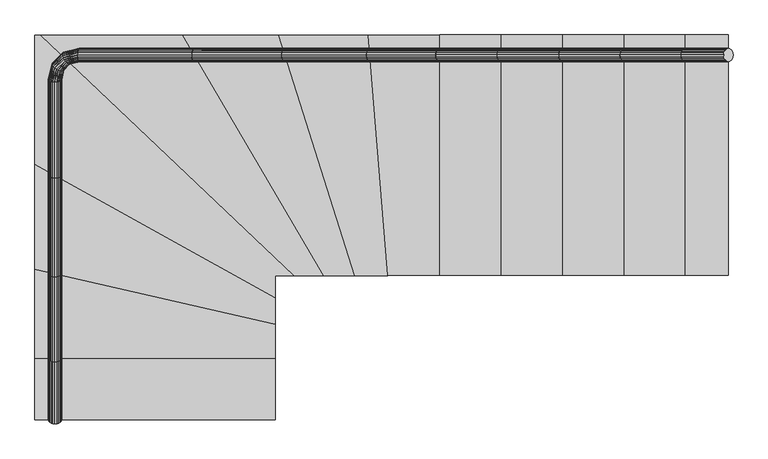
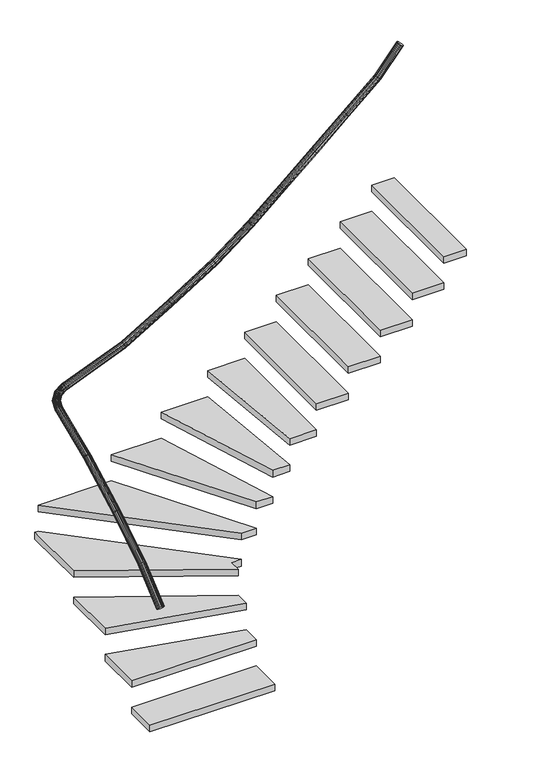
"""IFC4 building model written with IfcOpenShell, lengths in millimetres: stair geometry, 0_3d."""

import ifcopenshell
import ifcopenshell.guid

model = None  # the IFC model being written
_history = None  # IfcOwnerHistory: only IFC2X3 demands one
_inside = {}  # id of a spatial element -> (the spatial element, [elements in it])
_under = {}  # id of a project, library or spatial element -> (it, [spatial elements below it])
_declared = {}  # id of a project -> (the project, [libraries it declares])
_typed = {}  # id of a type object -> (the type object, [elements of that type])
_made_of = {}  # id of a material, layer set ... -> (it, [elements and type objects made of it])


def new_model(schema):
    """Start an empty IFC model of exactly this schema.

    Asked for "IFC4X3", IfcOpenShell would pick the latest addendum, in which some entities
    have other attributes; the version numbers below select the first issue.
    IFC2X3 requires an IfcOwnerHistory on every rooted entity: one is made here for all.
    """
    global model, _history
    if schema == "IFC4X3":
        model = ifcopenshell.file(schema_version=(4, 3, 0, 0))
    else:
        model = ifcopenshell.file(schema=schema)
    _inside.clear()
    _under.clear()
    _declared.clear()
    _typed.clear()
    _made_of.clear()
    _history = None
    if model.schema == "IFC2X3":
        org = make("IfcOrganization", Name="unknown")
        user = make(
            "IfcPersonAndOrganization",
            ThePerson=make("IfcPerson", FamilyName="unknown"),
            TheOrganization=org,
        )
        app = make(
            "IfcApplication",
            ApplicationDeveloper=org,
            Version="unknown",
            ApplicationFullName="unknown",
            ApplicationIdentifier="unknown",
        )
        _history = make(
            "IfcOwnerHistory",
            OwningUser=user,
            OwningApplication=app,
            ChangeAction="ADDED",
            CreationDate=0,
        )
    return model


def make(cls, **values):
    """One entity of the class cls with the attributes given. An attribute that is None is left unset."""
    return model.create_entity(
        cls, **{name: value for name, value in values.items() if value is not None}
    )


def rooted(cls, **values):
    """An entity with a GlobalId (a new one), such as an element, a storey or a relation."""
    return make(cls, GlobalId=ifcopenshell.guid.new(), OwnerHistory=_history, **values)


def si_unit(unit_type, name, prefix=None):
    """IfcSIUnit, for example si_unit("LENGTHUNIT", "METRE", prefix="MILLI")."""
    return make("IfcSIUnit", UnitType=unit_type, Prefix=prefix, Name=name)


def assignment(units):
    """IfcUnitAssignment: the units of a project."""
    return None if units is None else make("IfcUnitAssignment", Units=units)


def point(xyz):
    """IfcCartesianPoint."""
    return None if xyz is None else make("IfcCartesianPoint", Coordinates=xyz)


def direction(xyz):
    """IfcDirection."""
    return None if xyz is None else make("IfcDirection", DirectionRatios=xyz)


def frame(location, z_axis=None, x_axis=None):
    """IfcAxis2Placement3D, a coordinate frame: its origin and axes. An axis left out is left unset."""
    return make(
        "IfcAxis2Placement3D",
        Location=point(location),
        Axis=direction(z_axis),
        RefDirection=direction(x_axis),
    )


def origin():
    """The frame at (0, 0, 0) with its axes left unset."""
    return frame((0.0, 0.0, 0.0))


def origin_with_axes():
    """The frame at (0, 0, 0) with the z axis (0, 0, 1) and the x axis (1, 0, 0) written out."""
    return frame((0.0, 0.0, 0.0), z_axis=(0.0, 0.0, 1.0), x_axis=(1.0, 0.0, 0.0))


def place(relative_to, where):
    """IfcLocalPlacement: puts the frame where relative to a parent placement (None: the world)."""
    return make(
        "IfcLocalPlacement", PlacementRelTo=relative_to, RelativePlacement=where
    )


def context(
    kind, dimensions, precision=None, world=None, true_north=None, identifier=None
):
    """IfcGeometricRepresentationContext, for example the 3D "Model" context."""
    return make(
        "IfcGeometricRepresentationContext",
        ContextIdentifier=identifier,
        ContextType=kind,
        CoordinateSpaceDimension=dimensions,
        Precision=precision,
        WorldCoordinateSystem=world,
        TrueNorth=true_north,
    )


def project(units=None, contexts=None):
    """IfcProject with its units and contexts."""
    return rooted(
        "IfcProject",
        Name="project",
        RepresentationContexts=contexts,
        UnitsInContext=assignment(units),
    )


def spatial(cls, under=None, at=None, **own):
    """A site, building, storey or space (cls), placed at a placement, below another one or the project."""
    s = rooted(cls, ObjectPlacement=at, **own)
    if under is not None:
        _under.setdefault(under.id(), (under, []))[1].append(s)
    return s


def polyline(points):
    """IfcPolyline through the points."""
    return make("IfcPolyline", Points=[point(p) for p in points])


def outline(outer, holes=None, kind="AREA"):
    """IfcArbitraryClosedProfileDef: a profile drawn as a closed curve; with holes, ...WithVoids."""
    if holes is None:
        return make("IfcArbitraryClosedProfileDef", ProfileType=kind, OuterCurve=outer)
    return make(
        "IfcArbitraryProfileDefWithVoids",
        ProfileType=kind,
        OuterCurve=outer,
        InnerCurves=holes,
    )


def extrude(swept, where, along, depth):
    """IfcExtrudedAreaSolid: the profile swept, set in the frame where, extruded along a direction by depth."""
    return make(
        "IfcExtrudedAreaSolid",
        SweptArea=swept,
        Position=where,
        ExtrudedDirection=direction(along),
        Depth=depth,
    )


def faces_of(points, faces, orient=None, outer=None):
    """IfcFace entities. A face is a list of loops; a loop is a list of indices into points, from 0.

    orient and outer hold one flag for each loop. By default every Orientation is true, the
    first loop of a face is its IfcFaceOuterBound and the others are IfcFaceBound.
    """
    made = []
    for i, loops in enumerate(faces):
        bounds = []
        for j, loop in enumerate(loops):
            is_outer = j == 0 if outer is None else outer[i][j]
            bounds.append(
                make(
                    "IfcFaceOuterBound" if is_outer else "IfcFaceBound",
                    Bound=make("IfcPolyLoop", Polygon=[points[k] for k in loop]),
                    Orientation=True if orient is None else orient[i][j],
                )
            )
        made.append(make("IfcFace", Bounds=bounds))
    return made


def faceted_brep(points, faces, orient=None, outer=None, voids=None):
    """IfcFacetedBrep: a solid bounded by flat faces; with voids (closed shells), ...WithVoids."""
    shared = [point(p) for p in points]
    hull = make("IfcClosedShell", CfsFaces=faces_of(shared, faces, orient, outer))
    if voids is None:
        return make("IfcFacetedBrep", Outer=hull)
    return make(
        "IfcFacetedBrepWithVoids",
        Outer=hull,
        Voids=[
            make(cls, CfsFaces=faces_of(shared, fs, o, b)) for cls, fs, o, b in voids
        ],
    )


def shape(context_of_items, identifier, shape_type, items):
    """IfcShapeRepresentation: the items that make up one representation, for example the "Body"."""
    return make(
        "IfcShapeRepresentation",
        ContextOfItems=context_of_items,
        RepresentationIdentifier=identifier,
        RepresentationType=shape_type,
        Items=items,
    )


def source(mapping_origin, context_of_items, identifier, shape_type, items):
    """IfcRepresentationMap: a shape defined once, which mapped items show again and again."""
    return make(
        "IfcRepresentationMap",
        MappingOrigin=mapping_origin,
        MappedRepresentation=shape(context_of_items, identifier, shape_type, items),
    )


def transform(
    local_origin,
    x_axis=None,
    y_axis=None,
    z_axis=None,
    scale=None,
    scale2=None,
    scale3=None,
    uniform=True,
):
    """IfcCartesianTransformationOperator3D, or its non-uniform kind. x_axis, y_axis, z_axis: its Axis1, 2, 3."""
    if uniform:
        return make(
            "IfcCartesianTransformationOperator3D",
            Axis1=direction(x_axis),
            Axis2=direction(y_axis),
            LocalOrigin=point(local_origin),
            Scale=scale,
            Axis3=direction(z_axis),
        )
    return make(
        "IfcCartesianTransformationOperator3DnonUniform",
        Axis1=direction(x_axis),
        Axis2=direction(y_axis),
        LocalOrigin=point(local_origin),
        Scale=scale,
        Axis3=direction(z_axis),
        Scale2=scale2,
        Scale3=scale3,
    )


def mapped(mapping_source, mapping_target):
    """IfcMappedItem: shows the shape of a source again, moved by a transform."""
    return make(
        "IfcMappedItem", MappingSource=mapping_source, MappingTarget=mapping_target
    )


def made_of(thing, what):
    """Note that an element or type object is made of a material, layer set ...; save() writes the relation."""
    if what is not None:
        _made_of.setdefault(what.id(), (what, []))[1].append(thing)
    return thing


def element(
    cls,
    number,
    at=None,
    inside=None,
    cuts=None,
    type_object=None,
    material=None,
    context=None,
    identifier="Body",
    shape_type=None,
    held_by="IfcProductDefinitionShape",
    body=None,
    shapes=None,
    **own,
):
    """One element of the class cls, such as IfcWall. Its Tag is "e" and its number.

    at: its placement. inside: the storey or other place that contains it. cuts: it is an
    opening in that element (IfcRelVoidsElement). A single representation is given by context,
    identifier, shape_type and body (its items); several are given by shapes. held_by: the class
    of the entity that holds the representations. save() writes the other relations.
    """
    e = rooted(cls, Tag="e%d" % number, ObjectPlacement=at, **own)
    if body is not None:
        shapes = [shape(context, identifier, shape_type, body)]
    if shapes is not None:
        e.Representation = make(held_by, Representations=shapes)
    if inside is not None:
        _inside.setdefault(inside.id(), (inside, []))[1].append(e)
    if cuts is not None:
        rooted(
            "IfcRelVoidsElement", RelatingBuildingElement=cuts, RelatedOpeningElement=e
        )
    if type_object is not None:
        _typed.setdefault(type_object.id(), (type_object, []))[1].append(e)
    return made_of(e, material)


def aggregate(whole, parts):
    """IfcRelAggregates: a whole, such as a stair, and the parts it consists of."""
    return rooted("IfcRelAggregates", RelatingObject=whole, RelatedObjects=parts)


def save(model, path):
    """Write the relations noted so far, then the file.

    IfcRelAggregates (storeys below a building ...), IfcRelContainedInSpatialStructure (elements
    in a storey), IfcRelDefinesByType, IfcRelAssociatesMaterial and IfcRelDeclares: one each for
    every whole, place, type object, material and project.
    """
    for whole, parts in _under.values():
        aggregate(whole, parts)
    for where, things in _inside.values():
        rooted(
            "IfcRelContainedInSpatialStructure",
            RelatedElements=things,
            RelatingStructure=where,
        )
    for kind, things in _typed.values():
        rooted("IfcRelDefinesByType", RelatedObjects=things, RelatingType=kind)
    for what, things in _made_of.values():
        rooted("IfcRelAssociatesMaterial", RelatedObjects=things, RelatingMaterial=what)
    for by, libraries in _declared.values():
        rooted("IfcRelDeclares", RelatingContext=by, RelatedDefinitions=libraries)
    model.write(path)


def stair_5edd69db(model_context):
    return source(origin(), model_context, "Body", "SolidModel", [
        faceted_brep([(98.7764129, 932.7420558, 1514.6204637), (100.0, 929.684358, 1521.0), (98.7764129, 926.6266602, 1527.3795363), (95.2254249, 923.8682712, 1533.1345992), (89.6946313, 921.6792012, 1537.7018429), (82.7254249, 920.2737318, 1540.6341939), (75.0, 919.7894401, 1541.6446132), (67.2745751, 920.2737318, 1540.6341939), (60.3053687, 921.6792012, 1537.7018429), (54.7745751, 923.8682712, 1533.1345992), (51.2235871, 926.6266602, 1527.3795363), (50.0, 929.684358, 1521.0), (51.2235871, 932.7420558, 1514.6204637), (54.7745751, 935.5004448, 1508.8654008), (60.3053687, 937.6895148, 1504.2981571), (67.2745751, 939.0949842, 1501.3658061), (75.0, 939.5792759, 1500.3553868), (82.7254249, 939.0949842, 1501.3658061), (89.6946313, 937.6895148, 1504.2981571), (95.2254249, 935.5004448, 1508.8654008), (98.7764129, 1285.0513301, 1677.6833099), (100.0, 1287.7837588, 1671.1673734), (98.7764129, 1290.5161874, 1664.651437), (95.2254249, 1292.9811469, 1658.7733258), (89.6946313, 1294.9373498, 1654.1084303), (82.7254249, 1296.1933094, 1651.1133831), (75.0, 1296.6260836, 1650.0813601), (67.2745751, 1296.1933094, 1651.1133831), (60.3053687, 1294.9373498, 1654.1084303), (54.7745751, 1292.9811469, 1658.7733258), (51.2235871, 1290.5161874, 1664.651437), (50.0, 1287.7837588, 1671.1673734), (51.2235871, 1285.0513301, 1677.6833099), (54.7745751, 1282.5863706, 1683.5614211), (60.3053687, 1280.6301677, 1688.2263166), (67.2745751, 1279.3742081, 1691.2213638), (75.0, 1278.9414339, 1692.2533868), (82.7254249, 1279.3742081, 1691.2213638), (89.6946313, 1280.6301677, 1688.2263166), (95.2254249, 1282.5863706, 1683.5614211)], [[[0, 1, 2, 3, 4, 5, 6, 7, 8, 9, 10, 11, 12, 13, 14, 15, 16, 17, 18, 19]], [[20, 21, 22, 23, 24, 25, 26, 27, 28, 29, 30, 31, 32, 33, 34, 35, 36, 37, 38, 39]], [[2, 1, 21, 20]], [[3, 2, 20, 39]], [[4, 3, 39, 38]], [[5, 4, 38, 37]], [[6, 5, 37, 36]], [[7, 6, 36, 35]], [[8, 7, 35, 34]], [[9, 8, 34, 33]], [[10, 9, 33, 32]], [[11, 10, 32, 31]], [[12, 11, 31, 30]], [[13, 12, 30, 29]], [[14, 13, 29, 28]], [[15, 14, 28, 27]], [[16, 15, 27, 26]], [[17, 16, 26, 25]], [[18, 17, 25, 24]], [[19, 18, 24, 23]], [[0, 19, 23, 22]], [[1, 0, 22, 21]]]),
        faceted_brep([(98.7764129, 1290.5161874, 1664.651437), (100.0, 1287.7837588, 1671.1673734), (98.7764129, 1285.0513301, 1677.6833099), (95.2254249, 1282.5863706, 1683.5614211), (89.6946313, 1280.6301677, 1688.2263166), (82.7254249, 1279.3742081, 1691.2213638), (75.0, 1278.9414339, 1692.2533868), (67.2745751, 1279.3742081, 1691.2213638), (60.3053687, 1280.6301677, 1688.2263166), (54.7745751, 1282.5863706, 1683.5614211), (51.2235871, 1285.0513301, 1677.6833099), (50.0, 1287.7837588, 1671.1673734), (51.2235871, 1290.5161874, 1664.651437), (54.7745751, 1292.9811469, 1658.7733258), (60.3053687, 1294.9373498, 1654.1084303), (67.2745751, 1296.1933094, 1651.1133831), (75.0, 1296.6260836, 1650.0813601), (82.7254249, 1296.1933094, 1651.1133831), (89.6946313, 1294.9373498, 1654.1084303), (95.2254249, 1292.9811469, 1658.7733258), (108.4537582, 1324.5154276, 1696.3642542), (105.7104032, 1322.0507015, 1702.5140419), (101.0887593, 1321.0018856, 1708.0618455), (95.041225, 1321.4716452, 1712.4646074), (88.1597753, 1323.4139971, 1715.2913546), (81.1180142, 1326.6388103, 1716.2653852), (74.6052386, 1330.8304176, 1715.2913546), (69.2589642, 1335.5785152, 1712.4646074), (65.6025216, 1340.4183264, 1708.0618455), (63.9938289, 1344.8760967, 1702.5140419), (64.5903561, 1348.5154683, 1696.3642542), (67.333711, 1350.9801944, 1690.2144665), (71.955355, 1352.0290104, 1684.6666629), (78.0028893, 1351.5592507, 1680.263901), (84.884339, 1349.6168988, 1677.4371539), (91.9261001, 1346.3920857, 1676.4631232), (98.4388757, 1342.2004784, 1677.4371539), (103.7851501, 1337.4523807, 1680.263901), (107.4415927, 1332.6125695, 1684.6666629), (109.0502854, 1328.1547993, 1690.2144665), (130.5571891, 1346.5425346, 1722.9446322), (126.94301, 1345.9702551, 1729.1115573), (122.5136876, 1347.6039425, 1734.6748208), (117.7027948, 1351.2836802, 1739.0898518), (112.9812552, 1356.6492697, 1741.9244761), (108.8129654, 1363.1772042, 1742.897081), (105.6009573, 1370.2235085, 1741.9244761), (103.6646338, 1377.1034167, 1739.0898518), (103.1918166, 1383.1417611, 1734.6748208), (104.2287884, 1387.7474664, 1729.1115573), (106.6740431, 1390.4696941, 1722.9446322), (110.2882222, 1391.0419735, 1716.7777071), (114.7175446, 1389.4082861, 1711.2144436), (119.5284374, 1385.7285485, 1706.7994126), (124.249977, 1380.362959, 1703.9647883), (128.4183865, 1373.8351437, 1702.9918937), (131.6302749, 1366.7887202, 1703.9647883), (133.5665984, 1359.908812, 1706.7994126), (134.0394156, 1353.8704676, 1711.2144436), (133.0024438, 1349.2647623, 1716.7777071), (167.5717581, 1355.003504, 1747.6562732), (164.9242456, 1356.2270911, 1754.2071717), (162.53589, 1359.7780791, 1760.1168226), (160.6404803, 1365.3088727, 1764.8067482), (159.4235524, 1372.2780791, 1767.8178657), (159.0042276, 1380.003504, 1768.8554261), (159.4235524, 1387.7289288, 1767.8178657), (160.6404803, 1394.6981353, 1764.8067482), (162.53589, 1400.2289288, 1760.1168226), (164.9242456, 1403.7799169, 1754.2071717), (167.5717581, 1405.003504, 1747.6562732), (170.2192707, 1403.7799169, 1741.1053746), (172.6076263, 1400.2289288, 1735.1957237), (174.503036, 1394.6981353, 1730.5057981), (175.7199639, 1387.7289288, 1727.4946806), (176.1392887, 1380.003504, 1726.4571202), (175.7199639, 1372.2780791, 1727.4946806), (174.503036, 1365.3088727, 1730.5057981), (172.6076263, 1359.7780791, 1735.1957237), (170.2192707, 1356.2270911, 1741.1053746), (593.3502688, 1356.2270911, 1927.3533843), (596.4865027, 1355.003504, 1921.0), (599.6227367, 1356.2270911, 1914.6466157), (602.4519742, 1359.7780791, 1908.915145), (604.6972697, 1365.3088727, 1904.3666241), (606.1388383, 1372.2780791, 1901.4462938), (606.6355689, 1380.003504, 1900.4400166), (606.1388383, 1387.7289288, 1901.4462938), (604.6972697, 1394.6981353, 1904.3666241), (602.4519742, 1400.2289288, 1908.915145), (599.6227367, 1403.7799169, 1914.6466157), (596.4865027, 1405.003504, 1921.0), (593.3502688, 1403.7799169, 1927.3533843), (590.5210313, 1400.2289288, 1933.084855), (588.2757357, 1394.6981353, 1937.6333759), (586.8341672, 1387.7289288, 1940.5537062), (586.3374366, 1380.003504, 1941.5599834), (586.8341672, 1372.2780791, 1940.5537062), (588.2757357, 1365.3088727, 1937.6333759), (590.5210313, 1359.7780791, 1933.084855)], [[[0, 1, 2, 3, 4, 5, 6, 7, 8, 9, 10, 11, 12, 13, 14, 15, 16, 17, 18, 19]], [[2, 1, 20]], [[21, 2, 20]], [[3, 2, 21]], [[22, 3, 21]], [[4, 3, 22]], [[23, 4, 22]], [[5, 4, 23]], [[24, 5, 23]], [[6, 5, 24]], [[25, 6, 24]], [[7, 6, 25]], [[26, 7, 25]], [[8, 7, 26]], [[27, 8, 26]], [[9, 8, 27]], [[28, 9, 27]], [[10, 9, 28]], [[29, 10, 28]], [[11, 10, 29]], [[30, 11, 29]], [[12, 11, 30]], [[31, 12, 30]], [[13, 12, 31]], [[32, 13, 31]], [[14, 13, 32]], [[33, 14, 32]], [[15, 14, 33]], [[34, 15, 33]], [[16, 15, 34]], [[35, 16, 34]], [[17, 16, 35]], [[36, 17, 35]], [[18, 17, 36]], [[37, 18, 36]], [[19, 18, 37]], [[38, 19, 37]], [[0, 19, 38]], [[39, 0, 38]], [[1, 0, 39]], [[20, 1, 39]], [[21, 20, 40]], [[41, 21, 40]], [[22, 21, 41]], [[42, 22, 41]], [[23, 22, 42]], [[43, 23, 42]], [[24, 23, 43]], [[44, 24, 43]], [[25, 24, 44]], [[26, 25, 44, 45]], [[46, 26, 45]], [[27, 26, 46]], [[47, 27, 46]], [[28, 27, 47]], [[48, 28, 47]], [[29, 28, 48]], [[49, 29, 48]], [[30, 29, 49]], [[50, 30, 49]], [[31, 30, 50]], [[51, 31, 50]], [[32, 31, 51]], [[52, 32, 51]], [[33, 32, 52]], [[53, 33, 52]], [[34, 33, 53]], [[54, 34, 53]], [[35, 34, 54]], [[36, 35, 54, 55]], [[56, 36, 55]], [[37, 36, 56]], [[57, 37, 56]], [[38, 37, 57]], [[58, 38, 57]], [[39, 38, 58]], [[59, 39, 58]], [[20, 39, 59]], [[40, 20, 59]], [[41, 40, 60]], [[61, 41, 60]], [[42, 41, 61]], [[62, 42, 61]], [[43, 42, 62]], [[63, 43, 62]], [[44, 43, 63]], [[64, 44, 63]], [[45, 44, 64]], [[65, 45, 64]], [[46, 45, 65]], [[66, 46, 65]], [[47, 46, 66]], [[67, 47, 66]], [[48, 47, 67]], [[68, 48, 67]], [[49, 48, 68]], [[69, 49, 68]], [[50, 49, 69]], [[70, 50, 69]], [[51, 50, 70]], [[71, 51, 70]], [[52, 51, 71]], [[72, 52, 71]], [[53, 52, 72]], [[73, 53, 72]], [[54, 53, 73]], [[74, 54, 73]], [[55, 54, 74]], [[75, 55, 74]], [[56, 55, 75]], [[76, 56, 75]], [[57, 56, 76]], [[77, 57, 76]], [[58, 57, 77]], [[78, 58, 77]], [[59, 58, 78]], [[79, 59, 78]], [[40, 59, 79]], [[60, 40, 79]], [[80, 81, 82, 83, 84, 85, 86, 87, 88, 89, 90, 91, 92, 93, 94, 95, 96, 97, 98, 99]], [[61, 60, 81, 80]], [[62, 61, 80, 99]], [[63, 62, 99, 98]], [[64, 63, 98, 97]], [[65, 64, 97, 96]], [[66, 65, 96, 95]], [[67, 66, 95, 94]], [[68, 67, 94, 93]], [[69, 68, 93, 92]], [[70, 69, 92, 91]], [[71, 70, 91, 90]], [[72, 71, 90, 89]], [[73, 72, 89, 88]], [[74, 73, 88, 87]], [[75, 74, 87, 86]], [[76, 75, 86, 85]], [[77, 76, 85, 84]], [[78, 77, 84, 83]], [[79, 78, 83, 82]], [[60, 79, 82, 81]]]),
        extrude(outline(polyline([(1247.8590327, 1455.003504), (1514.6018366, 1455.003504), (1514.6018366, 555.003504), (1321.3446405, 555.003504), (1247.8590327, 1455.003504)])), frame((0.0, 0.0, 1400.0), z_axis=(0.0, 0.0, 1.0), x_axis=(1.0, 0.0, 0.0)), (0.0, 0.0, 1.0), 50.0),
        faceted_brep([(2439.7169138, 1356.2270911, 3316.0845069), (2434.6018366, 1355.003504, 3321.0), (2429.4867594, 1356.2270911, 3325.9154931), (2424.8723816, 1359.7780791, 3330.3498235), (2421.2103906, 1365.3088727, 3333.8689281), (2418.8592477, 1372.2780791, 3336.1283323), (2418.049099, 1380.003504, 3336.9068699), (2418.8592477, 1387.7289288, 3336.1283323), (2421.2103906, 1394.6981353, 3333.8689281), (2424.8723816, 1400.2289288, 3330.3498235), (2429.4867594, 1403.7799169, 3325.9154931), (2434.6018366, 1405.003504, 3321.0), (2439.7169138, 1403.7799169, 3316.0845069), (2444.3312916, 1400.2289288, 3311.6501765), (2447.9932826, 1394.6981353, 3308.1310719), (2450.3444255, 1387.7289288, 3305.8716677), (2451.1545742, 1380.003504, 3305.0931301), (2450.3444255, 1372.2780791, 3305.8716677), (2447.9932826, 1365.3088727, 3308.1310719), (2444.3312916, 1359.7780791, 3311.6501765), (2589.488001, 1356.2270911, 3525.4205726), (2595.0, 1355.003504, 3521.0), (2600.511999, 1356.2270911, 3516.5794274), (2605.4844451, 1359.7780791, 3512.5915713), (2609.4306006, 1365.3088727, 3509.4267908), (2611.9641885, 1372.2780791, 3507.3948766), (2612.8372033, 1380.003504, 3506.6947267), (2611.9641885, 1387.7289288, 3507.3948766), (2609.4306006, 1394.6981353, 3509.4267908), (2605.4844451, 1400.2289288, 3512.5915713), (2600.511999, 1403.7799169, 3516.5794274), (2595.0, 1405.003504, 3521.0), (2589.488001, 1403.7799169, 3525.4205726), (2584.5155549, 1400.2289288, 3529.4084287), (2580.5693994, 1394.6981353, 3532.5732092), (2578.0358115, 1387.7289288, 3534.6051234), (2577.1627967, 1380.003504, 3535.3052733), (2578.0358115, 1372.2780791, 3534.6051234), (2580.5693994, 1365.3088727, 3532.5732092), (2584.5155549, 1359.7780791, 3529.4084287)], [[[0, 1, 2, 3, 4, 5, 6, 7, 8, 9, 10, 11, 12, 13, 14, 15, 16, 17, 18, 19]], [[20, 21, 22, 23, 24, 25, 26, 27, 28, 29, 30, 31, 32, 33, 34, 35, 36, 37, 38, 39]], [[2, 1, 21, 20]], [[3, 2, 20, 39]], [[4, 3, 39, 38]], [[5, 4, 38, 37]], [[6, 5, 37, 36]], [[7, 6, 36, 35]], [[8, 7, 35, 34]], [[9, 8, 34, 33]], [[10, 9, 33, 32]], [[11, 10, 32, 31]], [[12, 11, 31, 30]], [[13, 12, 30, 29]], [[14, 13, 29, 28]], [[15, 14, 28, 27]], [[16, 15, 27, 26]], [[17, 16, 26, 25]], [[18, 17, 25, 24]], [[19, 18, 24, 23]], [[0, 19, 23, 22]], [[1, 0, 22, 21]]]),
        extrude(outline(polyline([(1.2235871, -7.0656631), (0.0, 0.0), (1.2235871, 7.0656631), (4.7745751, 13.4396898), (10.3053687, 18.498146), (17.2745751, 21.7458748), (25.0, 22.864966), (32.7254248, 21.7458748), (39.6946313, 18.498146), (45.2254248, 13.4396898), (48.7764129, 7.0656631), (50.0, 0.0), (48.7764129, -7.0656631), (45.2254248, -13.4396898), (39.6946313, -18.498146), (32.7254248, -21.7458748), (25.0, -22.864966), (17.2745751, -21.7458748), (10.3053687, -18.498146), (4.7745751, -13.4396898), (1.2235871, -7.0656631)])), frame((1744.6018366, 1355.003504, 2721.0), z_axis=(0.7546055221637331, 0.0, 0.656178714924524), x_axis=(0.0, 1.0, 0.0)), (0.0, 0.0, 1.0), 304.7950131),
        extrude(outline(polyline([(0.0, 971.2987014), (0.0, 1455.003504), (22.6704161, 1455.003504), (970.0, 555.003504), (900.0, 555.003504), (900.0, 471.9265809), (0.0, 971.2987014)])), frame((0.0, 0.0, 600.0), z_axis=(0.0, 0.0, 1.0), x_axis=(1.0, 0.0, 0.0)), (0.0, 0.0, 1.0), 50.0),
        extrude(outline(polyline([(1744.6018366, 1455.003504), (1974.6018366, 1455.003504), (1974.6018366, 555.003504), (1744.6018366, 555.003504), (1744.6018366, 1455.003504)])), frame((0.0, 0.0, 1800.0), z_axis=(0.0, 0.0, 1.0), x_axis=(1.0, 0.0, 0.0)), (0.0, 0.0, 1.0), 50.0),
        extrude(outline(polyline([(0.0, 15.003504), (0.0, 245.003504), (900.0, 245.003504), (900.0, 15.003504), (0.0, 15.003504)])), origin_with_axes(), (0.0, 0.0, 1.0), 50.0),
        extrude(outline(polyline([(0.0, 245.003504), (0.0, 577.9706943), (900.0, 372.0363136), (900.0, 245.003504), (0.0, 245.003504)])), frame((0.0, 0.0, 200.0), z_axis=(0.0, 0.0, 1.0), x_axis=(1.0, 0.0, 0.0)), (0.0, 0.0, 1.0), 50.0),
        faceted_brep([(98.7764129, 249.2359946, 1115.3170403), (100.0, 245.003504, 1121.0), (98.7764129, 240.7710134, 1126.6829597), (95.2254249, 236.9528284, 1131.8096318), (89.6946313, 233.9226997, 1135.8781817), (82.7254249, 231.9772373, 1138.4903516), (75.0, 231.3068766, 1139.390444), (67.2745751, 231.9772373, 1138.4903516), (60.3053687, 233.9226997, 1135.8781817), (54.7745751, 236.9528284, 1131.8096318), (51.2235871, 240.7710134, 1126.6829597), (50.0, 245.003504, 1121.0), (51.2235871, 249.2359946, 1115.3170403), (54.7745751, 253.0541795, 1110.1903682), (60.3053687, 256.0843082, 1106.1218183), (67.2745751, 258.0297706, 1103.5096484), (75.0, 258.7001313, 1102.609556), (82.7254249, 258.0297706, 1103.5096484), (89.6946313, 256.0843082, 1106.1218183), (95.2254249, 253.0541795, 1110.1903682), (98.7764129, 557.2313341, 1327.0973463), (100.0, 560.8094959, 1321.0), (98.7764129, 564.3876578, 1314.9026537), (95.2254249, 567.6155643, 1309.4021582), (89.6946313, 570.1772453, 1305.0369402), (82.7254249, 571.8219458, 1302.2342978), (75.0, 572.388671, 1301.268573), (67.2745751, 571.8219458, 1302.2342978), (60.3053687, 570.1772453, 1305.0369402), (54.7745751, 567.6155643, 1309.4021582), (51.2235871, 564.3876578, 1314.9026537), (50.0, 560.8094959, 1321.0), (51.2235871, 557.2313341, 1327.0973463), (54.7745751, 554.0034276, 1332.5978418), (60.3053687, 551.4417465, 1336.9630598), (67.2745751, 549.797046, 1339.7657022), (75.0, 549.2303209, 1340.731427), (82.7254249, 549.797046, 1339.7657022), (89.6946313, 551.4417465, 1336.9630598), (95.2254249, 554.0034276, 1332.5978418)], [[[0, 1, 2, 3, 4, 5, 6, 7, 8, 9, 10, 11, 12, 13, 14, 15, 16, 17, 18, 19]], [[20, 21, 22, 23, 24, 25, 26, 27, 28, 29, 30, 31, 32, 33, 34, 35, 36, 37, 38, 39]], [[2, 1, 21, 20]], [[3, 2, 20, 39]], [[4, 3, 39, 38]], [[5, 4, 38, 37]], [[6, 5, 37, 36]], [[7, 6, 36, 35]], [[8, 7, 35, 34]], [[9, 8, 34, 33]], [[10, 9, 33, 32]], [[11, 10, 32, 31]], [[12, 11, 31, 30]], [[13, 12, 30, 29]], [[14, 13, 29, 28]], [[15, 14, 28, 27]], [[16, 15, 27, 26]], [[17, 16, 26, 25]], [[18, 17, 25, 24]], [[19, 18, 24, 23]], [[0, 19, 23, 22]], [[1, 0, 22, 21]]]),
        faceted_brep([(1258.0212623, 1356.2270911, 2315.1927019), (1253.9828334, 1355.003504, 2321.0), (1249.9444045, 1356.2270911, 2326.8072981), (1246.3012851, 1359.7780791, 2332.0461373), (1243.4100892, 1365.3088727, 2336.2037037), (1241.5538272, 1372.2780791, 2338.8730256), (1240.9142029, 1380.003504, 2339.7928113), (1241.5538272, 1387.7289288, 2338.8730256), (1243.4100892, 1394.6981353, 2336.2037037), (1246.3012851, 1400.2289288, 2332.0461373), (1249.9444045, 1403.7799169, 2326.8072981), (1253.9828334, 1405.003504, 2321.0), (1258.0212623, 1403.7799169, 2315.1927019), (1261.6643817, 1400.2289288, 2309.9538627), (1264.5555775, 1394.6981353, 2305.7962963), (1266.4118396, 1387.7289288, 2303.1269744), (1267.0514639, 1380.003504, 2302.2071887), (1266.4118396, 1372.2780791, 2303.1269744), (1264.5555775, 1365.3088727, 2305.7962963), (1261.6643817, 1359.7780791, 2309.9538627), (1510.1286941, 1356.2270911, 2526.4736972), (1514.6018366, 1355.003504, 2521.0), (1519.0749792, 1356.2270911, 2515.5263028), (1523.1102593, 1359.7780791, 2510.5884093), (1526.3126758, 1365.3088727, 2506.6696747), (1528.3687538, 1372.2780791, 2504.1536923), (1529.07723, 1380.003504, 2503.2867438), (1528.3687538, 1387.7289288, 2504.1536923), (1526.3126758, 1394.6981353, 2506.6696747), (1523.1102593, 1400.2289288, 2510.5884093), (1519.0749792, 1403.7799169, 2515.5263028), (1514.6018366, 1405.003504, 2521.0), (1510.1286941, 1403.7799169, 2526.4736972), (1506.0934139, 1400.2289288, 2531.4115907), (1502.8909974, 1394.6981353, 2535.3303253), (1500.8349194, 1387.7289288, 2537.8463077), (1500.1264432, 1380.003504, 2538.7132562), (1500.8349194, 1372.2780791, 2537.8463077), (1502.8909974, 1365.3088727, 2535.3303253), (1506.0934139, 1359.7780791, 2531.4115907)], [[[0, 1, 2, 3, 4, 5, 6, 7, 8, 9, 10, 11, 12, 13, 14, 15, 16, 17, 18, 19]], [[20, 21, 22, 23, 24, 25, 26, 27, 28, 29, 30, 31, 32, 33, 34, 35, 36, 37, 38, 39]], [[2, 1, 21, 20]], [[3, 2, 20, 39]], [[4, 3, 39, 38]], [[5, 4, 38, 37]], [[6, 5, 37, 36]], [[7, 6, 36, 35]], [[8, 7, 35, 34]], [[9, 8, 34, 33]], [[10, 9, 33, 32]], [[11, 10, 32, 31]], [[12, 11, 31, 30]], [[13, 12, 30, 29]], [[14, 13, 29, 28]], [[15, 14, 28, 27]], [[16, 15, 27, 26]], [[17, 16, 26, 25]], [[18, 17, 25, 24]], [[19, 18, 24, 23]], [[0, 19, 23, 22]], [[1, 0, 22, 21]]]),
        extrude(outline(polyline([(911.6691967, 1455.003504), (1247.8590327, 1455.003504), (1321.3446405, 555.003504), (1197.5344765, 555.003504), (911.6691967, 1455.003504)])), frame((0.0, 0.0, 1200.0), z_axis=(0.0, 0.0, 1.0), x_axis=(1.0, 0.0, 0.0)), (0.0, 0.0, 1.0), 50.0),
        extrude(outline(polyline([(1514.6018366, 1455.003504), (1744.6018366, 1455.003504), (1744.6018366, 555.003504), (1514.6018366, 555.003504), (1514.6018366, 1455.003504)])), frame((0.0, 0.0, 1600.0), z_axis=(0.0, 0.0, 1.0), x_axis=(1.0, 0.0, 0.0)), (0.0, 0.0, 1.0), 50.0),
        extrude(outline(polyline([(1.2235871, -7.0656631), (0.0, 0.0), (1.2235871, 7.0656631), (4.7745751, 13.4396898), (10.3053687, 18.498146), (17.2745751, 21.7458748), (25.0, 22.864966), (32.7254248, 21.7458748), (39.6946313, 18.498146), (45.2254248, 13.4396898), (48.7764129, 7.0656631), (50.0, 0.0), (48.7764129, -7.0656631), (45.2254248, -13.4396898), (39.6946313, -18.498146), (32.7254248, -21.7458748), (25.0, -22.864966), (17.2745751, -21.7458748), (10.3053687, -18.498146), (4.7745751, -13.4396898), (1.2235871, -7.0656631)])), frame((1974.6018366, 1355.003504, 2921.0), z_axis=(0.7546055221637457, 0.0, 0.6561787149245096), x_axis=(0.0, 1.0, 0.0)), (0.0, 0.0, 1.0), 304.7950131),
        faceted_brep([(939.1658894, 1356.2270911, 2114.9642231), (935.4913033, 1355.003504, 2121.0), (931.8167172, 1356.2270911, 2127.0357769), (928.5018253, 1359.7780791, 2132.4807298), (925.8711121, 1365.3088727, 2136.801869), (924.1820903, 1372.2780791, 2139.5762111), (923.600093, 1380.003504, 2140.5321843), (924.1820903, 1387.7289288, 2139.5762111), (925.8711121, 1394.6981353, 2136.801869), (928.5018253, 1400.2289288, 2132.4807298), (931.8167172, 1403.7799169, 2127.0357769), (935.4913033, 1405.003504, 2121.0), (939.1658894, 1403.7799169, 2114.9642231), (942.4807814, 1400.2289288, 2109.5192702), (945.1114946, 1394.6981353, 2105.198131), (946.8005164, 1387.7289288, 2102.4237889), (947.3825136, 1380.003504, 2101.4678157), (946.8005164, 1372.2780791, 2102.4237889), (945.1114946, 1365.3088727, 2105.198131), (942.4807814, 1359.7780791, 2109.5192702), (1249.9444045, 1356.2270911, 2326.8072981), (1253.9828334, 1355.003504, 2321.0), (1258.0212623, 1356.2270911, 2315.1927019), (1261.6643817, 1359.7780791, 2309.9538627), (1264.5555775, 1365.3088727, 2305.7962963), (1266.4118396, 1372.2780791, 2303.1269744), (1267.0514639, 1380.003504, 2302.2071887), (1266.4118396, 1387.7289288, 2303.1269744), (1264.5555775, 1394.6981353, 2305.7962963), (1261.6643817, 1400.2289288, 2309.9538627), (1258.0212623, 1403.7799169, 2315.1927019), (1253.9828334, 1405.003504, 2321.0), (1249.9444045, 1403.7799169, 2326.8072981), (1246.3012851, 1400.2289288, 2332.0461373), (1243.4100892, 1394.6981353, 2336.2037037), (1241.5538272, 1387.7289288, 2338.8730256), (1240.9142029, 1380.003504, 2339.7928113), (1241.5538272, 1372.2780791, 2338.8730256), (1243.4100892, 1365.3088727, 2336.2037037), (1246.3012851, 1359.7780791, 2332.0461373)], [[[0, 1, 2, 3, 4, 5, 6, 7, 8, 9, 10, 11, 12, 13, 14, 15, 16, 17, 18, 19]], [[20, 21, 22, 23, 24, 25, 26, 27, 28, 29, 30, 31, 32, 33, 34, 35, 36, 37, 38, 39]], [[2, 1, 21, 20]], [[3, 2, 20, 39]], [[4, 3, 39, 38]], [[5, 4, 38, 37]], [[6, 5, 37, 36]], [[7, 6, 36, 35]], [[8, 7, 35, 34]], [[9, 8, 34, 33]], [[10, 9, 33, 32]], [[11, 10, 32, 31]], [[12, 11, 31, 30]], [[13, 12, 30, 29]], [[14, 13, 29, 28]], [[15, 14, 28, 27]], [[16, 15, 27, 26]], [[17, 16, 26, 25]], [[18, 17, 25, 24]], [[19, 18, 24, 23]], [[0, 19, 23, 22]], [[1, 0, 22, 21]]]),
        extrude(outline(polyline([(2434.6018366, 1455.003504), (2595.0, 1455.003504), (2595.0, 555.003504), (2434.6018366, 555.003504), (2434.6018366, 1455.003504)])), frame((0.0, 0.0, 2400.0), z_axis=(0.0, 0.0, 1.0), x_axis=(1.0, 0.0, 0.0)), (0.0, 0.0, 1.0), 50.0),
        faceted_brep([(98.7764129, 564.3876578, 1314.9026537), (100.0, 560.8094959, 1321.0), (98.7764129, 557.2313341, 1327.0973463), (95.2254249, 554.0034276, 1332.5978418), (89.6946313, 551.4417465, 1336.9630598), (82.7254249, 549.797046, 1339.7657022), (75.0, 549.2303209, 1340.731427), (67.2745751, 549.797046, 1339.7657022), (60.3053687, 551.4417465, 1336.9630598), (54.7745751, 554.0034276, 1332.5978418), (51.2235871, 557.2313341, 1327.0973463), (50.0, 560.8094959, 1321.0), (51.2235871, 564.3876578, 1314.9026537), (54.7745751, 567.6155643, 1309.4021582), (60.3053687, 570.1772453, 1305.0369402), (67.2745751, 571.8219458, 1302.2342978), (75.0, 572.388671, 1301.268573), (82.7254249, 571.8219458, 1302.2342978), (89.6946313, 570.1772453, 1305.0369402), (95.2254249, 567.6155643, 1309.4021582), (98.7764129, 926.6266602, 1527.3795363), (100.0, 929.684358, 1521.0), (98.7764129, 932.7420558, 1514.6204637), (95.2254249, 935.5004448, 1508.8654008), (89.6946313, 937.6895148, 1504.2981571), (82.7254249, 939.0949842, 1501.3658061), (75.0, 939.5792759, 1500.3553868), (67.2745751, 939.0949842, 1501.3658061), (60.3053687, 937.6895148, 1504.2981571), (54.7745751, 935.5004448, 1508.8654008), (51.2235871, 932.7420558, 1514.6204637), (50.0, 929.684358, 1521.0), (51.2235871, 926.6266602, 1527.3795363), (54.7745751, 923.8682712, 1533.1345992), (60.3053687, 921.6792012, 1537.7018429), (67.2745751, 920.2737318, 1540.6341939), (75.0, 919.7894401, 1541.6446132), (82.7254249, 920.2737318, 1540.6341939), (89.6946313, 921.6792012, 1537.7018429), (95.2254249, 923.8682712, 1533.1345992)], [[[0, 1, 2, 3, 4, 5, 6, 7, 8, 9, 10, 11, 12, 13, 14, 15, 16, 17, 18, 19]], [[20, 21, 22, 23, 24, 25, 26, 27, 28, 29, 30, 31, 32, 33, 34, 35, 36, 37, 38, 39]], [[2, 1, 21, 20]], [[3, 2, 20, 39]], [[4, 3, 39, 38]], [[5, 4, 38, 37]], [[6, 5, 37, 36]], [[7, 6, 36, 35]], [[8, 7, 35, 34]], [[9, 8, 34, 33]], [[10, 9, 33, 32]], [[11, 10, 32, 31]], [[12, 11, 31, 30]], [[13, 12, 30, 29]], [[14, 13, 29, 28]], [[15, 14, 28, 27]], [[16, 15, 27, 26]], [[17, 16, 26, 25]], [[18, 17, 25, 24]], [[19, 18, 24, 23]], [[0, 19, 23, 22]], [[1, 0, 22, 21]]]),
        faceted_brep([(599.6227367, 1356.2270911, 1914.6466157), (596.4865027, 1355.003504, 1921.0), (593.3502688, 1356.2270911, 1927.3533843), (590.5210313, 1359.7780791, 1933.084855), (588.2757357, 1365.3088727, 1937.6333759), (586.8341672, 1372.2780791, 1940.5537062), (586.3374366, 1380.003504, 1941.5599834), (586.8341672, 1387.7289288, 1940.5537062), (588.2757357, 1394.6981353, 1937.6333759), (590.5210313, 1400.2289288, 1933.084855), (593.3502688, 1403.7799169, 1927.3533843), (596.4865027, 1405.003504, 1921.0), (599.6227367, 1403.7799169, 1914.6466157), (602.4519742, 1400.2289288, 1908.915145), (604.6972697, 1394.6981353, 1904.3666241), (606.1388383, 1387.7289288, 1901.4462938), (606.6355689, 1380.003504, 1900.4400166), (606.1388383, 1372.2780791, 1901.4462938), (604.6972697, 1365.3088727, 1904.3666241), (602.4519742, 1359.7780791, 1908.915145), (931.8167172, 1356.2270911, 2127.0357769), (935.4913033, 1355.003504, 2121.0), (939.1658894, 1356.2270911, 2114.9642231), (942.4807814, 1359.7780791, 2109.5192702), (945.1114946, 1365.3088727, 2105.198131), (946.8005164, 1372.2780791, 2102.4237889), (947.3825136, 1380.003504, 2101.4678157), (946.8005164, 1387.7289288, 2102.4237889), (945.1114946, 1394.6981353, 2105.198131), (942.4807814, 1400.2289288, 2109.5192702), (939.1658894, 1403.7799169, 2114.9642231), (935.4913033, 1405.003504, 2121.0), (931.8167172, 1403.7799169, 2127.0357769), (928.5018253, 1400.2289288, 2132.4807298), (925.8711121, 1394.6981353, 2136.801869), (924.1820903, 1387.7289288, 2139.5762111), (923.600093, 1380.003504, 2140.5321843), (924.1820903, 1372.2780791, 2139.5762111), (925.8711121, 1365.3088727, 2136.801869), (928.5018253, 1359.7780791, 2132.4807298)], [[[0, 1, 2, 3, 4, 5, 6, 7, 8, 9, 10, 11, 12, 13, 14, 15, 16, 17, 18, 19]], [[20, 21, 22, 23, 24, 25, 26, 27, 28, 29, 30, 31, 32, 33, 34, 35, 36, 37, 38, 39]], [[2, 1, 21, 20]], [[3, 2, 20, 39]], [[4, 3, 39, 38]], [[5, 4, 38, 37]], [[6, 5, 37, 36]], [[7, 6, 36, 35]], [[8, 7, 35, 34]], [[9, 8, 34, 33]], [[10, 9, 33, 32]], [[11, 10, 32, 31]], [[12, 11, 31, 30]], [[13, 12, 30, 29]], [[14, 13, 29, 28]], [[15, 14, 28, 27]], [[16, 15, 27, 26]], [[17, 16, 26, 25]], [[18, 17, 25, 24]], [[19, 18, 24, 23]], [[0, 19, 23, 22]], [[1, 0, 22, 21]]]),
        extrude(outline(polyline([(0.0, 577.9706943), (0.0, 971.2987014), (900.0, 471.9265809), (900.0, 372.0363136), (0.0, 577.9706943)])), frame((0.0, 0.0, 400.0), z_axis=(0.0, 0.0, 1.0), x_axis=(1.0, 0.0, 0.0)), (0.0, 0.0, 1.0), 50.0),
        faceted_brep([(2209.2381743, 1356.2270911, 3115.6682116), (2204.6018366, 1355.003504, 3121.0), (2199.9654989, 1356.2270911, 3126.3317884), (2195.7829982, 1359.7780791, 3131.1416641), (2192.4637469, 1365.3088727, 3134.9588031), (2190.3326564, 1372.2780791, 3137.4095572), (2189.5983326, 1380.003504, 3138.2540296), (2190.3326564, 1387.7289288, 3137.4095572), (2192.4637469, 1394.6981353, 3134.9588031), (2195.7829982, 1400.2289288, 3131.1416641), (2199.9654989, 1403.7799169, 3126.3317884), (2204.6018366, 1405.003504, 3121.0), (2209.2381743, 1403.7799169, 3115.6682116), (2213.420675, 1400.2289288, 3110.8583359), (2216.7399263, 1394.6981353, 3107.0411969), (2218.8710168, 1387.7289288, 3104.5904428), (2219.6053406, 1380.003504, 3103.7459704), (2218.8710168, 1372.2780791, 3104.5904428), (2216.7399263, 1365.3088727, 3107.0411969), (2213.420675, 1359.7780791, 3110.8583359), (2429.4867594, 1356.2270911, 3325.9154931), (2434.6018366, 1355.003504, 3321.0), (2439.7169138, 1356.2270911, 3316.0845069), (2444.3312916, 1359.7780791, 3311.6501765), (2447.9932826, 1365.3088727, 3308.1310719), (2450.3444255, 1372.2780791, 3305.8716677), (2451.1545742, 1380.003504, 3305.0931301), (2450.3444255, 1387.7289288, 3305.8716677), (2447.9932826, 1394.6981353, 3308.1310719), (2444.3312916, 1400.2289288, 3311.6501765), (2439.7169138, 1403.7799169, 3316.0845069), (2434.6018366, 1405.003504, 3321.0), (2429.4867594, 1403.7799169, 3325.9154931), (2424.8723816, 1400.2289288, 3330.3498235), (2421.2103906, 1394.6981353, 3333.8689281), (2418.8592477, 1387.7289288, 3336.1283323), (2418.049099, 1380.003504, 3336.9068699), (2418.8592477, 1372.2780791, 3336.1283323), (2421.2103906, 1365.3088727, 3333.8689281), (2424.8723816, 1359.7780791, 3330.3498235)], [[[0, 1, 2, 3, 4, 5, 6, 7, 8, 9, 10, 11, 12, 13, 14, 15, 16, 17, 18, 19]], [[20, 21, 22, 23, 24, 25, 26, 27, 28, 29, 30, 31, 32, 33, 34, 35, 36, 37, 38, 39]], [[2, 1, 21, 20]], [[3, 2, 20, 39]], [[4, 3, 39, 38]], [[5, 4, 38, 37]], [[6, 5, 37, 36]], [[7, 6, 36, 35]], [[8, 7, 35, 34]], [[9, 8, 34, 33]], [[10, 9, 33, 32]], [[11, 10, 32, 31]], [[12, 11, 31, 30]], [[13, 12, 30, 29]], [[14, 13, 29, 28]], [[15, 14, 28, 27]], [[16, 15, 27, 26]], [[17, 16, 26, 25]], [[18, 17, 25, 24]], [[19, 18, 24, 23]], [[0, 19, 23, 22]], [[1, 0, 22, 21]]]),
        extrude(outline(polyline([(552.4387223, 1455.003504), (911.6691967, 1455.003504), (1197.5344765, 555.003504), (1081.0120874, 555.003504), (552.4387223, 1455.003504)])), frame((0.0, 0.0, 1000.0), z_axis=(0.0, 0.0, 1.0), x_axis=(1.0, 0.0, 0.0)), (0.0, 0.0, 1.0), 50.0),
        extrude(outline(polyline([(2204.6018366, 1455.003504), (2434.6018366, 1455.003504), (2434.6018366, 555.003504), (2204.6018366, 555.003504), (2204.6018366, 1455.003504)])), frame((0.0, 0.0, 2200.0), z_axis=(0.0, 0.0, 1.0), x_axis=(1.0, 0.0, 0.0)), (0.0, 0.0, 1.0), 50.0),
        faceted_brep([(1519.0749792, 1356.2270911, 2515.5263028), (1514.6018366, 1355.003504, 2521.0), (1510.1286941, 1356.2270911, 2526.4736972), (1506.0934139, 1359.7780791, 2531.4115907), (1502.8909974, 1365.3088727, 2535.3303253), (1500.8349194, 1372.2780791, 2537.8463077), (1500.1264432, 1380.003504, 2538.7132562), (1500.8349194, 1387.7289288, 2537.8463077), (1502.8909974, 1394.6981353, 2535.3303253), (1506.0934139, 1400.2289288, 2531.4115907), (1510.1286941, 1403.7799169, 2526.4736972), (1514.6018366, 1405.003504, 2521.0), (1519.0749792, 1403.7799169, 2515.5263028), (1523.1102593, 1400.2289288, 2510.5884093), (1526.3126758, 1394.6981353, 2506.6696747), (1528.3687538, 1387.7289288, 2504.1536923), (1529.07723, 1380.003504, 2503.2867438), (1528.3687538, 1372.2780791, 2504.1536923), (1526.3126758, 1365.3088727, 2506.6696747), (1523.1102593, 1359.7780791, 2510.5884093), (1739.9654989, 1356.2270911, 2726.3317884), (1744.6018366, 1355.003504, 2721.0), (1749.2381743, 1356.2270911, 2715.6682116), (1753.420675, 1359.7780791, 2710.8583359), (1756.7399263, 1365.3088727, 2707.0411969), (1758.8710168, 1372.2780791, 2704.5904428), (1759.6053406, 1380.003504, 2703.7459704), (1758.8710168, 1387.7289288, 2704.5904428), (1756.7399263, 1394.6981353, 2707.0411969), (1753.420675, 1400.2289288, 2710.8583359), (1749.2381743, 1403.7799169, 2715.6682116), (1744.6018366, 1405.003504, 2721.0), (1739.9654989, 1403.7799169, 2726.3317884), (1735.7829982, 1400.2289288, 2731.1416641), (1732.4637469, 1394.6981353, 2734.9588031), (1730.3326564, 1387.7289288, 2737.4095572), (1729.5983326, 1380.003504, 2738.2540296), (1730.3326564, 1372.2780791, 2737.4095572), (1732.4637469, 1365.3088727, 2734.9588031), (1735.7829982, 1359.7780791, 2731.1416641)], [[[0, 1, 2, 3, 4, 5, 6, 7, 8, 9, 10, 11, 12, 13, 14, 15, 16, 17, 18, 19]], [[20, 21, 22, 23, 24, 25, 26, 27, 28, 29, 30, 31, 32, 33, 34, 35, 36, 37, 38, 39]], [[2, 1, 21, 20]], [[3, 2, 20, 39]], [[4, 3, 39, 38]], [[5, 4, 38, 37]], [[6, 5, 37, 36]], [[7, 6, 36, 35]], [[8, 7, 35, 34]], [[9, 8, 34, 33]], [[10, 9, 33, 32]], [[11, 10, 32, 31]], [[12, 11, 31, 30]], [[13, 12, 30, 29]], [[14, 13, 29, 28]], [[15, 14, 28, 27]], [[16, 15, 27, 26]], [[17, 16, 26, 25]], [[18, 17, 25, 24]], [[19, 18, 24, 23]], [[0, 19, 23, 22]], [[1, 0, 22, 21]]]),
        extrude(outline(polyline([(1974.6018366, 1455.003504), (2204.6018366, 1455.003504), (2204.6018366, 555.003504), (1974.6018366, 555.003504), (1974.6018366, 1455.003504)])), frame((0.0, 0.0, 2000.0), z_axis=(0.0, 0.0, 1.0), x_axis=(1.0, 0.0, 0.0)), (0.0, 0.0, 1.0), 50.0),
        faceted_brep([(98.7764129, 19.6398417, 915.6682116), (100.0, 15.003504, 921.0), (98.7764129, 10.3671663, 926.3317884), (95.2254249, 6.1846656, 931.1416641), (89.6946313, 2.8654143, 934.9588031), (82.7254249, 0.7343238, 937.4095572), (75.0, 0.0, 938.2540296), (67.2745751, 0.7343238, 937.4095572), (60.3053687, 2.8654143, 934.9588031), (54.7745751, 6.1846656, 931.1416641), (51.2235871, 10.3671663, 926.3317884), (50.0, 15.003504, 921.0), (51.2235871, 19.6398417, 915.6682116), (54.7745751, 23.8223423, 910.8583359), (60.3053687, 27.1415936, 907.0411969), (67.2745751, 29.2726842, 904.5904428), (75.0, 30.0070079, 903.7459704), (82.7254249, 29.2726842, 904.5904428), (89.6946313, 27.1415936, 907.0411969), (95.2254249, 23.8223423, 910.8583359), (98.7764129, 240.7710134, 1126.6829597), (100.0, 245.003504, 1121.0), (98.7764129, 249.2359946, 1115.3170403), (95.2254249, 253.0541795, 1110.1903682), (89.6946313, 256.0843082, 1106.1218183), (82.7254249, 258.0297706, 1103.5096484), (75.0, 258.7001313, 1102.609556), (67.2745751, 258.0297706, 1103.5096484), (60.3053687, 256.0843082, 1106.1218183), (54.7745751, 253.0541795, 1110.1903682), (51.2235871, 249.2359946, 1115.3170403), (50.0, 245.003504, 1121.0), (51.2235871, 240.7710134, 1126.6829597), (54.7745751, 236.9528284, 1131.8096318), (60.3053687, 233.9226997, 1135.8781817), (67.2745751, 231.9772373, 1138.4903516), (75.0, 231.3068766, 1139.390444), (82.7254249, 231.9772373, 1138.4903516), (89.6946313, 233.9226997, 1135.8781817), (95.2254249, 236.9528284, 1131.8096318)], [[[0, 1, 2, 3, 4, 5, 6, 7, 8, 9, 10, 11, 12, 13, 14, 15, 16, 17, 18, 19]], [[20, 21, 22, 23, 24, 25, 26, 27, 28, 29, 30, 31, 32, 33, 34, 35, 36, 37, 38, 39]], [[2, 1, 21, 20]], [[3, 2, 20, 39]], [[4, 3, 39, 38]], [[5, 4, 38, 37]], [[6, 5, 37, 36]], [[7, 6, 36, 35]], [[8, 7, 35, 34]], [[9, 8, 34, 33]], [[10, 9, 33, 32]], [[11, 10, 32, 31]], [[12, 11, 31, 30]], [[13, 12, 30, 29]], [[14, 13, 29, 28]], [[15, 14, 28, 27]], [[16, 15, 27, 26]], [[17, 16, 26, 25]], [[18, 17, 25, 24]], [[19, 18, 24, 23]], [[0, 19, 23, 22]], [[1, 0, 22, 21]]]),
        extrude(outline(polyline([(22.6704161, 1455.003504), (552.4387223, 1455.003504), (1081.0120874, 555.003504), (970.0, 555.003504), (22.6704161, 1455.003504)])), frame((0.0, 0.0, 800.0), z_axis=(0.0, 0.0, 1.0), x_axis=(1.0, 0.0, 0.0)), (0.0, 0.0, 1.0), 50.0),
    ])


if __name__ == "__main__":
    model = new_model("IFC4")
    model_context = context("Model", 3, world=origin())
    ifc_project = project(units=[si_unit("LENGTHUNIT", "METRE", prefix="MILLI")], contexts=[model_context])
    site = spatial("IfcSite", under=ifc_project)
    building = spatial("IfcBuilding", under=site)
    placement = place(None, origin())
    stair_shape = stair_5edd69db(model_context)
    element("IfcStair", 1, ObjectType="0_3d", at=placement, inside=building, context=model_context, shape_type="MappedRepresentation", body=[
        mapped(stair_shape, transform((0.0, 0.0, 0.0), x_axis=(1.0, 0.0, 0.0), y_axis=(0.0, 1.0, 0.0), z_axis=(0.0, 0.0, 1.0))),
    ])
    save(model, "model.ifc")

# Revit data of these elements
# Element 1 (IfcStair, "0_3d")
#   Materials on its faces: "*1", "weiss"
# Materials
#   "*1": class "Unassigned", colour RGB 175 175 175, transparency 0
#   "weiss": class "Unassigned", colour RGB 255 255 255, transparency 0
